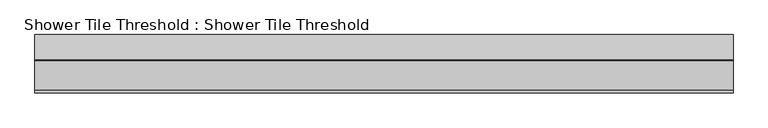
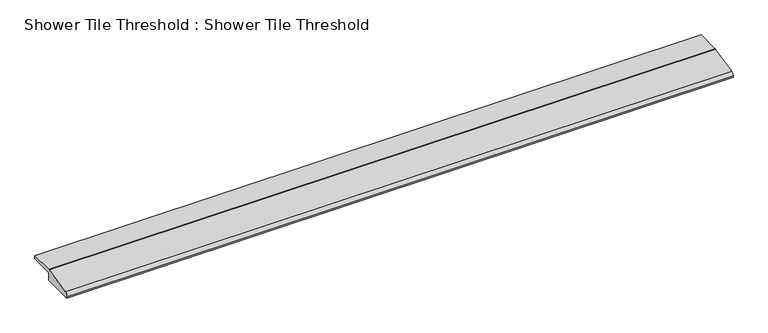
"""IFC4 building model written with IfcOpenShell, lengths in millimetres: proxy geometry, Shower Tile Threshold : Shower Tile Threshold."""

from ifc_helpers import new_model, si_unit, point, frame, frame_2d, origin, place, context, project, spatial, polyline, circle_curve, trimmed, segment, composite_curve, outline, extrude, source, transform, mapped, element, save


def shower_tile_threshold_shower_tile_threshold_c9caed11(model_context):
    return source(origin(), model_context, "Body", "SweptSolid", [
        extrude(outline(composite_curve([segment(polyline([(-95.25, -20.6375), (-152.4, -20.6375), (-152.4, -17.7937897)]), True, "CONTINUOUS"), segment(trimmed(circle_curve(frame_2d((-146.05, -17.7937897)), 6.35), [point((-152.4, -17.7937897))], [point((-147.4275084, -11.5950019))], False, "CARTESIAN"), True, "CONTINUOUS"), segment(polyline([(-147.4275084, -11.5950019), (-95.9304548, -0.1512122)]), True, "CONTINUOUS"), segment(trimmed(circle_curve(frame_2d((-94.5529463, -6.35)), 6.35), [point((-95.9304548, -0.1512122))], [point((-94.5529463, 0.0))], False, "CARTESIAN"), True, "CONTINUOUS"), segment(polyline([(-94.5529463, 0.0), (-50.8, 0.0), (-50.8, -6.35), (-95.25, -6.35), (-95.25, -20.6375)]), True, "CONTINUOUS")], self_intersect=False)), frame((-914.4, 0.0, 0.0), z_axis=(1.0, 0.0, 0.0), x_axis=(0.0, 1.0, 0.0)), (0.0, 0.0, 1.0), 1219.2),
    ])


if __name__ == "__main__":
    model = new_model("IFC4")
    model_context = context("Model", 3, world=origin())
    ifc_project = project(units=[si_unit("LENGTHUNIT", "METRE", prefix="MILLI")], contexts=[model_context])
    site = spatial("IfcSite", under=ifc_project)
    building = spatial("IfcBuilding", under=site)
    placement = place(None, origin())
    shower_tile_threshold_shower_tile_threshold_shape = shower_tile_threshold_shower_tile_threshold_c9caed11(model_context)
    element("IfcBuildingElementProxy", 1, Name="Shower Tile Threshold : Shower Tile Threshold", ObjectType="Shower Tile Threshold : Shower Tile Threshold", at=placement, inside=building, context=model_context, shape_type="MappedRepresentation", body=[
        mapped(shower_tile_threshold_shower_tile_threshold_shape, transform((0.0, 0.0, 0.0), x_axis=(1.0, 0.0, 0.0), y_axis=(0.0, 1.0, 0.0), z_axis=(0.0, 0.0, 1.0))),
    ])
    save(model, "model.ifc")

# Revit data of these elements
# Type "Shower Tile Threshold : Shower Tile Threshold"
#   Width [instance default] = 2' - 0"
#   Offset [instance default] = 0' - 1"
#   Material = Tile, Porcelain
# Element 1 (IfcBuildingElementProxy, "Shower Tile Threshold : Shower Tile Threshold")
#   Width = 4' - 0"
#   Offset = 0' - 0.53229"
# Materials
#   "Tile, Porcelain": class "Generic", colour RGB 119 125 134, transparency 0, Description = "Porcelain tile, 4\", white", Cost = 0
